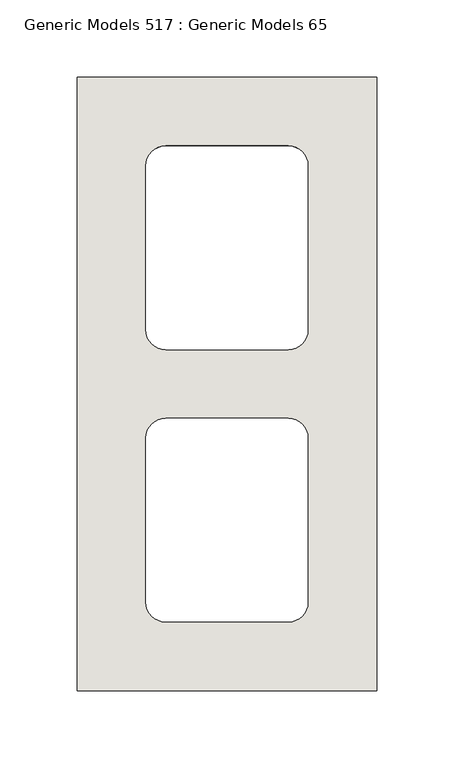
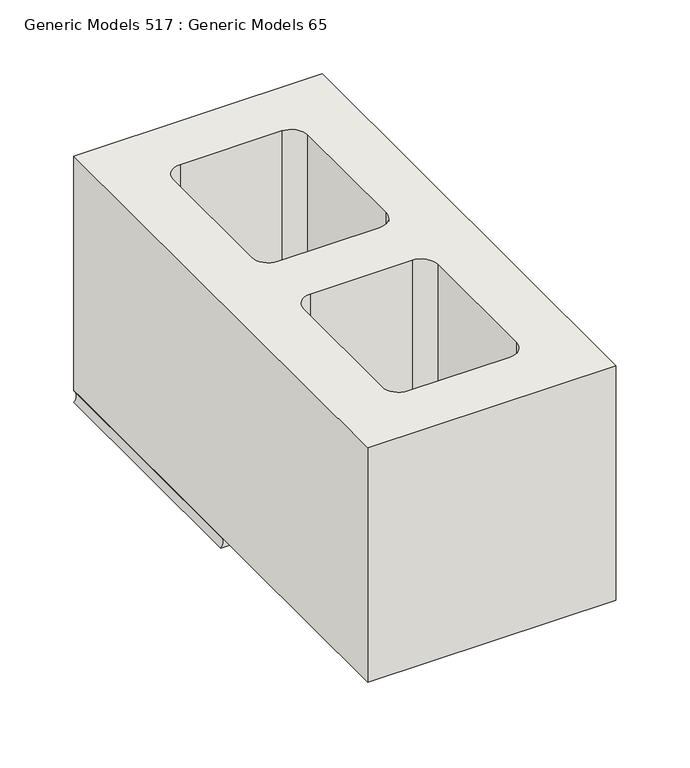
"""IFC4 building model written with IfcOpenShell, lengths in millimetres: wall geometry, Generic Models 517 : Generic Models 65."""

from ifc_helpers import new_model, si_unit, point, frame, frame_2d, origin, place, context, project, spatial, polyline, circle_curve, trimmed, segment, composite_curve, outline, extrude, source, transform, mapped, element, save
from ifc_brep_helpers import plane_surface, revolved_surface, advanced_brep


def generic_models_517_generic_models_65_be858529(model_context):
    return source(origin(), model_context, "Body", "SolidModel", [
        advanced_brep(
        [(428979.0125, 503.2375, 619.125), (428785.3375, 503.2375, 619.125), (428785.3375, 503.2375, 609.6), (428979.0125, 503.2375, 609.6), (428979.0125, 701.675, 619.125), (428979.0125, 701.675, 609.6), (428785.3375, 701.675, 609.6), (428785.3375, 701.675, 619.125), (428934.5625, 538.1625, 619.125), (428921.8625, 525.4625, 619.125), (428842.4875, 525.4625, 619.125), (428829.7875, 538.1625, 619.125), (428829.7875, 644.525, 619.125), (428842.4875, 657.225, 619.125), (428921.8625, 657.225, 619.125), (428934.5625, 644.525, 619.125), (428921.8625, 525.4625, 609.6), (428934.5625, 538.1625, 609.6), (428842.4875, 525.4625, 609.6), (428829.7875, 538.1625, 609.6), (428829.7875, 644.525, 609.6), (428842.4875, 657.225, 609.6), (428921.8625, 657.225, 609.6), (428934.5625, 644.525, 609.6)],
        [
            (0, 1),
            (1, 2, circle_curve(frame((428780.4545028, 503.2375, 614.3625), z_axis=(0.0, 1.0, 0.0), x_axis=(1.0, 0.0, 0.0)), 6.8209287)),
            (2, 3),
            (3, 0, circle_curve(frame((428983.8954972, 503.2375, 614.3625), z_axis=(0.0, 1.0, 0.0), x_axis=(-1.0, 0.0, 0.0)), 6.8209287)),
            (4, 5, circle_curve(frame((428983.8954972, 701.675, 614.3625), z_axis=(0.0, -1.0, 0.0), x_axis=(-1.0, 0.0, 0.0)), 6.8209287)),
            (5, 6),
            (6, 7, circle_curve(frame((428780.4545028, 701.675, 614.3625), z_axis=(0.0, -1.0, 0.0), x_axis=(1.0, 0.0, 0.0)), 6.8209287)),
            (7, 4),
            (0, 4),
            (7, 1),
            (8, 9, circle_curve(frame((428921.8625, 538.1625, 619.125), z_axis=(0.0, 0.0, -1.0), x_axis=(-1.0, 0.0, 0.0)), 12.7)),
            (9, 10),
            (10, 11, circle_curve(frame((428842.4875, 538.1625, 619.125), z_axis=(0.0, 0.0, -1.0), x_axis=(-1.0, 0.0, 0.0)), 12.7)),
            (11, 12),
            (12, 13, circle_curve(frame((428842.4875, 644.525, 619.125), z_axis=(0.0, 0.0, -1.0), x_axis=(-1.0, 0.0, 0.0)), 12.7)),
            (13, 14),
            (14, 15, circle_curve(frame((428921.8625, 644.525, 619.125), z_axis=(0.0, 0.0, -1.0), x_axis=(-1.0, 0.0, 0.0)), 12.7)),
            (15, 8),
            (16, 9),
            (8, 17),
            (17, 16, circle_curve(frame((428921.8625, 538.1625, 609.6), z_axis=(0.0, 0.0, -1.0), x_axis=(-1.0, 0.0, 0.0)), 12.7)),
            (16, 18),
            (18, 10),
            (18, 19, circle_curve(frame((428842.4875, 538.1625, 609.6), z_axis=(0.0, 0.0, -1.0), x_axis=(-1.0, 0.0, 0.0)), 12.7)),
            (19, 11),
            (19, 20),
            (20, 12),
            (20, 21, circle_curve(frame((428842.4875, 644.525, 609.6), z_axis=(0.0, 0.0, -1.0), x_axis=(-1.0, 0.0, 0.0)), 12.7)),
            (21, 13),
            (21, 22),
            (22, 14),
            (22, 23, circle_curve(frame((428921.8625, 644.525, 609.6), z_axis=(0.0, 0.0, -1.0), x_axis=(-1.0, 0.0, 0.0)), 12.7)),
            (23, 15),
            (23, 17),
            (6, 2),
            (5, 3),
        ],
        [
            plane_surface(frame((428882.175, 503.2375, 619.521875), z_axis=(0.0, -1.0, 0.0), x_axis=(0.0, 0.0, 1.0))),
            plane_surface(frame((428882.175, 701.675, 619.521875), z_axis=(0.0, 1.0, 0.0), x_axis=(0.0, 0.0, 1.0))),
            plane_surface(frame((428979.0125, 503.2375, 619.125), z_axis=(0.0, 0.0, 1.0), x_axis=(0.0, 1.0, 0.0))),
            revolved_surface(polyline([(428909.1625, 538.1625, 619.125), (428909.1625, 538.1625, 609.6)]), (428921.8625, 538.1625, 803.275), (0.0, 0.0, 1.0)),
            plane_surface(frame((428842.4875, 525.4625, 803.275), z_axis=(0.0, 1.0, 0.0), x_axis=(0.0, 0.0, -1.0))),
            revolved_surface(polyline([(428829.7875, 538.1625, 619.125), (428829.7875, 538.1625, 609.6)]), (428842.4875, 538.1625, 803.275), (0.0, 0.0, 1.0)),
            plane_surface(frame((428829.7875, 644.525, 803.275), z_axis=(1.0, 0.0, 0.0), x_axis=(0.0, 0.0, -1.0))),
            revolved_surface(polyline([(428829.7875, 644.525, 619.125), (428829.7875, 644.525, 609.6)]), (428842.4875, 644.525, 803.275), (0.0, 0.0, 1.0)),
            plane_surface(frame((428921.8625, 657.225, 803.275), z_axis=(0.0, -1.0, 0.0), x_axis=(0.0, 0.0, -1.0))),
            revolved_surface(polyline([(428909.1625, 644.525, 619.125), (428909.1625, 644.525, 609.6)]), (428921.8625, 644.525, 803.275), (0.0, 0.0, 1.0)),
            plane_surface(frame((428934.5625, 538.1625, 803.275), z_axis=(-1.0, 0.0, 0.0), x_axis=(0.0, 0.0, -1.0))),
            revolved_surface(polyline([(428787.2754315, 701.675, 614.3625), (428787.2754315, 503.2375, 614.3625)]), (428780.4545028, 503.2375, 614.3625), (0.0, 1.0, 0.0)),
            plane_surface(frame((428785.3375, 503.2375, 609.6), z_axis=(0.0, 0.0, -1.0), x_axis=(0.0, 1.0, 0.0))),
            revolved_surface(polyline([(428977.07456850004, 701.675, 614.3625), (428977.07456850004, 503.2375, 614.3625)]), (428983.8954972, 503.2375, 614.3625), (0.0, 1.0, 0.0)),
        ],
        [
            (0, [[1, 2, 3, 4]]),
            (1, [[5, 6, 7, 8]]),
            (2, [[-1, 9, -8, 10], [11, 12, 13, 14, 15, 16, 17, 18]]),
            (3, [[19, -11, 20, 21]]),
            (4, [[-19, 22, 23, -12]]),
            (5, [[-23, 24, 25, -13]]),
            (6, [[-25, 26, 27, -14]]),
            (7, [[-27, 28, 29, -15]]),
            (8, [[-29, 30, 31, -16]]),
            (9, [[-31, 32, 33, -17]]),
            (10, [[-33, 34, -20, -18]]),
            (11, [[-2, -10, -7, 35]]),
            (12, [[-3, -35, -6, 36], [-21, -34, -32, -30, -28, -26, -24, -22]]),
            (13, [[-4, -36, -5, -9]]),
        ],
    ),
        extrude(outline(polyline([(428979.0125, 304.8), (428785.3375, 304.8), (428785.3375, 701.675), (428979.0125, 701.675), (428979.0125, 304.8)]), holes=[composite_curve([segment(polyline([(428934.5625, 538.1625), (428934.5625, 644.525)]), True, "CONTINUOUS"), segment(trimmed(circle_curve(frame_2d((428921.8625, 644.525)), 12.7), [point((428934.5625, 644.525))], [point((428921.8625, 657.225))], True, "CARTESIAN"), True, "CONTINUOUS"), segment(polyline([(428921.8625, 657.225), (428842.4875, 657.225)]), True, "CONTINUOUS"), segment(trimmed(circle_curve(frame_2d((428842.4875, 644.525)), 12.7), [point((428842.4875, 657.225))], [point((428829.7875, 644.525))], True, "CARTESIAN"), True, "CONTINUOUS"), segment(polyline([(428829.7875, 644.525), (428829.7875, 538.1625)]), True, "CONTINUOUS"), segment(trimmed(circle_curve(frame_2d((428842.4875, 538.1625)), 12.7), [point((428829.7875, 538.1625))], [point((428842.4875, 525.4625))], True, "CARTESIAN"), True, "CONTINUOUS"), segment(polyline([(428842.4875, 525.4625), (428921.8625, 525.4625)]), True, "CONTINUOUS"), segment(trimmed(circle_curve(frame_2d((428921.8625, 538.1625)), 12.7), [point((428921.8625, 525.4625))], [point((428934.5625, 538.1625))], True, "CARTESIAN"), True, "CONTINUOUS")], self_intersect=False), composite_curve([segment(polyline([(428829.7875, 468.3125), (428829.7875, 361.95)]), True, "CONTINUOUS"), segment(trimmed(circle_curve(frame_2d((428842.4875, 361.95)), 12.7), [point((428829.7875, 361.95))], [point((428842.4875, 349.25))], True, "CARTESIAN"), True, "CONTINUOUS"), segment(polyline([(428842.4875, 349.25), (428921.8625, 349.25)]), True, "CONTINUOUS"), segment(trimmed(circle_curve(frame_2d((428921.8625, 361.95)), 12.7), [point((428921.8625, 349.25))], [point((428934.5625, 361.95))], True, "CARTESIAN"), True, "CONTINUOUS"), segment(polyline([(428934.5625, 361.95), (428934.5625, 468.3125)]), True, "CONTINUOUS"), segment(trimmed(circle_curve(frame_2d((428921.8625, 468.3125)), 12.7), [point((428934.5625, 468.3125))], [point((428921.8625, 481.0125))], True, "CARTESIAN"), True, "CONTINUOUS"), segment(polyline([(428921.8625, 481.0125), (428842.4875, 481.0125)]), True, "CONTINUOUS"), segment(trimmed(circle_curve(frame_2d((428842.4875, 468.3125)), 12.7), [point((428842.4875, 481.0125))], [point((428829.7875, 468.3125))], True, "CARTESIAN"), True, "CONTINUOUS")], self_intersect=False)]), frame((0.0, 0.0, 619.125), z_axis=(0.0, 0.0, 1.0), x_axis=(1.0, 0.0, 0.0)), (0.0, 0.0, 1.0), 193.675),
    ])


if __name__ == "__main__":
    model = new_model("IFC4")
    model_context = context("Model", 3, world=origin())
    ifc_project = project(units=[si_unit("LENGTHUNIT", "METRE", prefix="MILLI")], contexts=[model_context])
    site = spatial("IfcSite", under=ifc_project)
    building = spatial("IfcBuilding", under=site)
    placement = place(None, origin())
    generic_models_517_generic_models_65_shape = generic_models_517_generic_models_65_be858529(model_context)
    element("IfcWall", 1, ObjectType="Generic Models 517 : Generic Models 65", at=placement, inside=building, context=model_context, shape_type="MappedRepresentation", body=[
        mapped(generic_models_517_generic_models_65_shape, transform((0.0, 0.0, 0.0), x_axis=(1.0, 0.0, 0.0), y_axis=(0.0, 1.0, 0.0), z_axis=(0.0, 0.0, 1.0))),
    ])
    save(model, "model.ifc")

# Revit data of these elements
# Element 1 (IfcWall, "Generic Models 517 : Generic Models 65")
#   Materials on its faces: "CMU (SEE 'WALL TAG' FOR SIZE)", "MORTAR JOINT"
# Materials
#   "CMU (SEE 'WALL TAG' FOR SIZE)": class "Masonry", colour RGB 203 203 199, transparency 0, Description = "Concrete masonry units", Cost = 0
#   "MORTAR JOINT": class "Generic", colour RGB 120 120 120, transparency 0, Cost = 0
